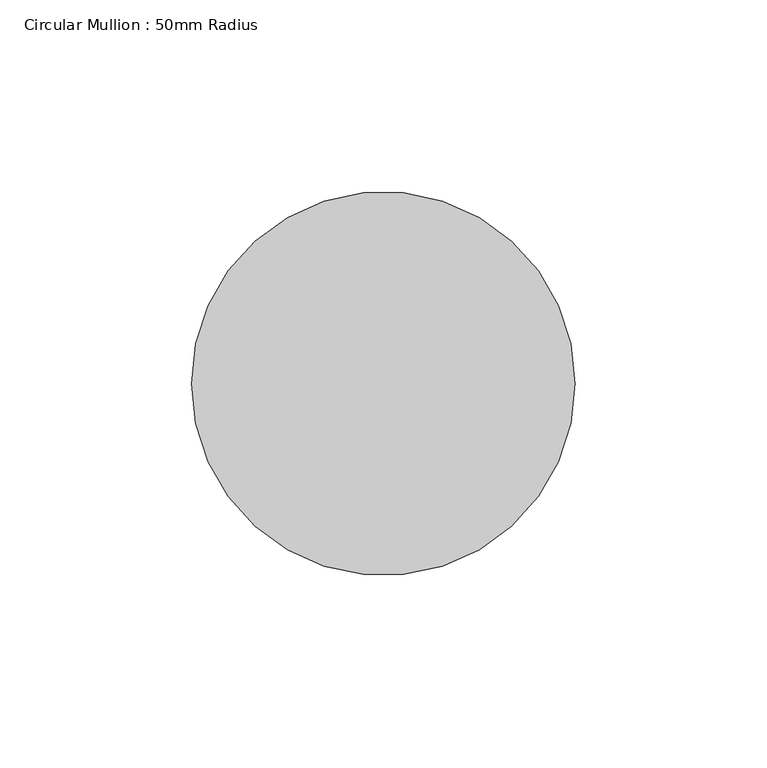
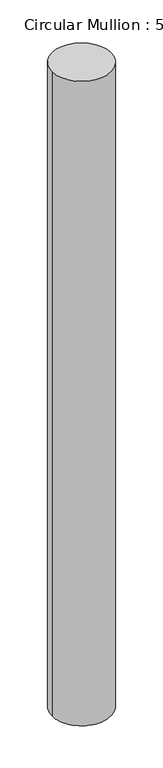
"""IFC4 building model written with IfcOpenShell, lengths in millimetres: member geometry, Circular Mullion : 50mm Radius."""

import ifcopenshell
import ifcopenshell.guid

model = None  # the IFC model being written
_history = None  # IfcOwnerHistory: only IFC2X3 demands one
_inside = {}  # id of a spatial element -> (the spatial element, [elements in it])
_under = {}  # id of a project, library or spatial element -> (it, [spatial elements below it])
_declared = {}  # id of a project -> (the project, [libraries it declares])
_typed = {}  # id of a type object -> (the type object, [elements of that type])
_made_of = {}  # id of a material, layer set ... -> (it, [elements and type objects made of it])


def new_model(schema):
    """Start an empty IFC model of exactly this schema.

    Asked for "IFC4X3", IfcOpenShell would pick the latest addendum, in which some entities
    have other attributes; the version numbers below select the first issue.
    IFC2X3 requires an IfcOwnerHistory on every rooted entity: one is made here for all.
    """
    global model, _history
    if schema == "IFC4X3":
        model = ifcopenshell.file(schema_version=(4, 3, 0, 0))
    else:
        model = ifcopenshell.file(schema=schema)
    _inside.clear()
    _under.clear()
    _declared.clear()
    _typed.clear()
    _made_of.clear()
    _history = None
    if model.schema == "IFC2X3":
        org = make("IfcOrganization", Name="unknown")
        user = make(
            "IfcPersonAndOrganization",
            ThePerson=make("IfcPerson", FamilyName="unknown"),
            TheOrganization=org,
        )
        app = make(
            "IfcApplication",
            ApplicationDeveloper=org,
            Version="unknown",
            ApplicationFullName="unknown",
            ApplicationIdentifier="unknown",
        )
        _history = make(
            "IfcOwnerHistory",
            OwningUser=user,
            OwningApplication=app,
            ChangeAction="ADDED",
            CreationDate=0,
        )
    return model


def make(cls, **values):
    """One entity of the class cls with the attributes given. An attribute that is None is left unset."""
    return model.create_entity(
        cls, **{name: value for name, value in values.items() if value is not None}
    )


def rooted(cls, **values):
    """An entity with a GlobalId (a new one), such as an element, a storey or a relation."""
    return make(cls, GlobalId=ifcopenshell.guid.new(), OwnerHistory=_history, **values)


def si_unit(unit_type, name, prefix=None):
    """IfcSIUnit, for example si_unit("LENGTHUNIT", "METRE", prefix="MILLI")."""
    return make("IfcSIUnit", UnitType=unit_type, Prefix=prefix, Name=name)


def assignment(units):
    """IfcUnitAssignment: the units of a project."""
    return None if units is None else make("IfcUnitAssignment", Units=units)


def point(xyz):
    """IfcCartesianPoint."""
    return None if xyz is None else make("IfcCartesianPoint", Coordinates=xyz)


def direction(xyz):
    """IfcDirection."""
    return None if xyz is None else make("IfcDirection", DirectionRatios=xyz)


def frame(location, z_axis=None, x_axis=None):
    """IfcAxis2Placement3D, a coordinate frame: its origin and axes. An axis left out is left unset."""
    return make(
        "IfcAxis2Placement3D",
        Location=point(location),
        Axis=direction(z_axis),
        RefDirection=direction(x_axis),
    )


def origin():
    """The frame at (0, 0, 0) with its axes left unset."""
    return frame((0.0, 0.0, 0.0))


def place(relative_to, where):
    """IfcLocalPlacement: puts the frame where relative to a parent placement (None: the world)."""
    return make(
        "IfcLocalPlacement", PlacementRelTo=relative_to, RelativePlacement=where
    )


def context(
    kind, dimensions, precision=None, world=None, true_north=None, identifier=None
):
    """IfcGeometricRepresentationContext, for example the 3D "Model" context."""
    return make(
        "IfcGeometricRepresentationContext",
        ContextIdentifier=identifier,
        ContextType=kind,
        CoordinateSpaceDimension=dimensions,
        Precision=precision,
        WorldCoordinateSystem=world,
        TrueNorth=true_north,
    )


def project(units=None, contexts=None):
    """IfcProject with its units and contexts."""
    return rooted(
        "IfcProject",
        Name="project",
        RepresentationContexts=contexts,
        UnitsInContext=assignment(units),
    )


def spatial(cls, under=None, at=None, **own):
    """A site, building, storey or space (cls), placed at a placement, below another one or the project."""
    s = rooted(cls, ObjectPlacement=at, **own)
    if under is not None:
        _under.setdefault(under.id(), (under, []))[1].append(s)
    return s


def ellipse_curve(where, semi_axis1, semi_axis2):
    """IfcEllipse in the frame where."""
    return make(
        "IfcEllipse", Position=where, SemiAxis1=semi_axis1, SemiAxis2=semi_axis2
    )


def shape(context_of_items, identifier, shape_type, items):
    """IfcShapeRepresentation: the items that make up one representation, for example the "Body"."""
    return make(
        "IfcShapeRepresentation",
        ContextOfItems=context_of_items,
        RepresentationIdentifier=identifier,
        RepresentationType=shape_type,
        Items=items,
    )


def source(mapping_origin, context_of_items, identifier, shape_type, items):
    """IfcRepresentationMap: a shape defined once, which mapped items show again and again."""
    return make(
        "IfcRepresentationMap",
        MappingOrigin=mapping_origin,
        MappedRepresentation=shape(context_of_items, identifier, shape_type, items),
    )


def transform(
    local_origin,
    x_axis=None,
    y_axis=None,
    z_axis=None,
    scale=None,
    scale2=None,
    scale3=None,
    uniform=True,
):
    """IfcCartesianTransformationOperator3D, or its non-uniform kind. x_axis, y_axis, z_axis: its Axis1, 2, 3."""
    if uniform:
        return make(
            "IfcCartesianTransformationOperator3D",
            Axis1=direction(x_axis),
            Axis2=direction(y_axis),
            LocalOrigin=point(local_origin),
            Scale=scale,
            Axis3=direction(z_axis),
        )
    return make(
        "IfcCartesianTransformationOperator3DnonUniform",
        Axis1=direction(x_axis),
        Axis2=direction(y_axis),
        LocalOrigin=point(local_origin),
        Scale=scale,
        Axis3=direction(z_axis),
        Scale2=scale2,
        Scale3=scale3,
    )


def mapped(mapping_source, mapping_target):
    """IfcMappedItem: shows the shape of a source again, moved by a transform."""
    return make(
        "IfcMappedItem", MappingSource=mapping_source, MappingTarget=mapping_target
    )


def made_of(thing, what):
    """Note that an element or type object is made of a material, layer set ...; save() writes the relation."""
    if what is not None:
        _made_of.setdefault(what.id(), (what, []))[1].append(thing)
    return thing


def element(
    cls,
    number,
    at=None,
    inside=None,
    cuts=None,
    type_object=None,
    material=None,
    context=None,
    identifier="Body",
    shape_type=None,
    held_by="IfcProductDefinitionShape",
    body=None,
    shapes=None,
    **own,
):
    """One element of the class cls, such as IfcWall. Its Tag is "e" and its number.

    at: its placement. inside: the storey or other place that contains it. cuts: it is an
    opening in that element (IfcRelVoidsElement). A single representation is given by context,
    identifier, shape_type and body (its items); several are given by shapes. held_by: the class
    of the entity that holds the representations. save() writes the other relations.
    """
    e = rooted(cls, Tag="e%d" % number, ObjectPlacement=at, **own)
    if body is not None:
        shapes = [shape(context, identifier, shape_type, body)]
    if shapes is not None:
        e.Representation = make(held_by, Representations=shapes)
    if inside is not None:
        _inside.setdefault(inside.id(), (inside, []))[1].append(e)
    if cuts is not None:
        rooted(
            "IfcRelVoidsElement", RelatingBuildingElement=cuts, RelatedOpeningElement=e
        )
    if type_object is not None:
        _typed.setdefault(type_object.id(), (type_object, []))[1].append(e)
    return made_of(e, material)


def aggregate(whole, parts):
    """IfcRelAggregates: a whole, such as a stair, and the parts it consists of."""
    return rooted("IfcRelAggregates", RelatingObject=whole, RelatedObjects=parts)


def save(model, path):
    """Write the relations noted so far, then the file.

    IfcRelAggregates (storeys below a building ...), IfcRelContainedInSpatialStructure (elements
    in a storey), IfcRelDefinesByType, IfcRelAssociatesMaterial and IfcRelDeclares: one each for
    every whole, place, type object, material and project.
    """
    for whole, parts in _under.values():
        aggregate(whole, parts)
    for where, things in _inside.values():
        rooted(
            "IfcRelContainedInSpatialStructure",
            RelatedElements=things,
            RelatingStructure=where,
        )
    for kind, things in _typed.values():
        rooted("IfcRelDefinesByType", RelatedObjects=things, RelatingType=kind)
    for what, things in _made_of.values():
        rooted("IfcRelAssociatesMaterial", RelatedObjects=things, RelatingMaterial=what)
    for by, libraries in _declared.values():
        rooted("IfcRelDeclares", RelatingContext=by, RelatedDefinitions=libraries)
    model.write(path)


def plane_surface(at):
    """IfcPlane: the flat surface through the origin of the frame at, square to its z axis."""
    return make("IfcPlane", Position=at)


def cylinder_surface(at, radius):
    """IfcCylindricalSurface: all points at the distance radius from the z axis of the frame at."""
    return make("IfcCylindricalSurface", Position=at, Radius=radius)


def advanced_brep(points, edges, surfaces, faces):
    """IfcAdvancedBrep: a solid bounded by faces that lie on surfaces and meet in shared edges.

    An edge is (start, end): straight between two places in points (the first is 0);
    or (start, end, curve); or (start, end, curve, False) where it runs against its curve.
    A face is (place in surfaces, loops), or (place, loops, False) where it looks against
    its surface's normal. A loop lists edges by number (the first is 1), with a minus sign
    where the edge is run from its end to its start. The first loop is the outer one.
    """
    corners = [point(p) for p in points]
    vertices = [make("IfcVertexPoint", VertexGeometry=c) for c in corners]
    made = []
    for start, end, *more in edges:
        made.append(
            make(
                "IfcEdgeCurve",
                EdgeStart=vertices[start],
                EdgeEnd=vertices[end],
                EdgeGeometry=more[0] if more else make("IfcPolyline", Points=[corners[start], corners[end]]),
                SameSense=more[1] if len(more) > 1 else True,
            )
        )
    hull = []
    for where, loops, *sense in faces:
        bounds = []
        for j, loop in enumerate(loops):
            ring = [make("IfcOrientedEdge", EdgeElement=made[abs(k) - 1], Orientation=k > 0) for k in loop]
            bounds.append(
                make(
                    "IfcFaceOuterBound" if j == 0 else "IfcFaceBound",
                    Bound=make("IfcEdgeLoop", EdgeList=ring),
                    Orientation=True,
                )
            )
        hull.append(make("IfcAdvancedFace", Bounds=bounds, FaceSurface=surfaces[where], SameSense=sense[0] if sense else True))
    return make("IfcAdvancedBrep", Outer=make("IfcClosedShell", CfsFaces=hull))


def circular_mullion_50mm_radius_71162de6(model_context):
    return source(origin(), model_context, "Body", "AdvancedBrep", [
        advanced_brep(
        [(-100.0, 0.0, 0.9449858), (0.0, 0.0, 0.0), (0.0, 0.0, -1144.6892863), (-100.0, 0.0, -1145.6702895)],
        [
            (0, 1, ellipse_curve(frame((-50.0, 0.0, 0.4724929), z_axis=(-0.009448458751315407, -0.014383764193855156, -0.9998519060115054), x_axis=(-0.548945231973302, -0.8356811391006849, 0.017209475446963905)), 50.0074058, 50.0)),
            (1, 2),
            (2, 3, ellipse_curve(frame((-50.0, 0.0, -1145.1797879), z_axis=(-0.009808466948255391, -0.014931818977067286, 0.9998404046437417), x_axis=(0.5489389174171557, 0.8356715262009603, 0.017865196383996137)), 50.007981, 50.0)),
            (3, 0),
            (1, 0, ellipse_curve(frame((-50.0, 0.0, 0.4724929), z_axis=(-0.009448458751315407, -0.014383764193855156, -0.9998519060115054), x_axis=(-0.548945231973302, -0.8356811391006849, 0.017209475446963905)), 50.0074058, 50.0)),
            (3, 2, ellipse_curve(frame((-50.0, 0.0, -1145.1797879), z_axis=(-0.009808466948255391, -0.014931818977067286, 0.9998404046437417), x_axis=(0.5489389174171557, 0.8356715262009603, 0.017865196383996137)), 50.007981, 50.0)),
        ],
        [
            cylinder_surface(frame((-50.0, 0.0, 0.0), z_axis=(0.0, 0.0, 1.0), x_axis=(1.0, 0.0, 0.0)), 50.0),
            plane_surface(frame((-254.7533386, 167.3432892, 0.0), z_axis=(0.009448458751315409, 0.01438376419385516, 0.9998519060115056), x_axis=(0.5489452319733018, 0.835681139100685, -0.017209475446966372))),
            plane_surface(frame((-254.7533386, 167.3432892, -1144.6892863), z_axis=(0.009808466948255393, 0.01493181897706729, -0.9998404046437419), x_axis=(0.5489389174171557, 0.8356715262009604, 0.01786519638400108))),
        ],
        [
            (0, [[1, 2, 3, 4]]),
            (0, [[5, -4, 6, -2]]),
            (1, [[-1, -5]]),
            (2, [[-6, -3]]),
        ],
    ),
    ])


if __name__ == "__main__":
    model = new_model("IFC4")
    model_context = context("Model", 3, world=origin())
    ifc_project = project(units=[si_unit("LENGTHUNIT", "METRE", prefix="MILLI")], contexts=[model_context])
    site = spatial("IfcSite", under=ifc_project)
    building = spatial("IfcBuilding", under=site)
    placement = place(None, origin())
    circular_mullion_50mm_radius_shape = circular_mullion_50mm_radius_71162de6(model_context)
    element("IfcMember", 1, ObjectType="Circular Mullion : 50mm Radius", at=placement, inside=building, context=model_context, shape_type="MappedRepresentation", body=[
        mapped(circular_mullion_50mm_radius_shape, transform((0.0, 0.0, 0.0), x_axis=(1.0, 0.0, 0.0), y_axis=(0.0, 1.0, 0.0), z_axis=(0.0, 0.0, 1.0))),
    ])
    save(model, "model.ifc")

# Revit data of these elements
# Type "Circular Mullion : 50mm Radius"
#   built-in parameter 1007350 = 0.164042 (stored number, unit not read)
# Element 1 (IfcMember, "Circular Mullion : 50mm Radius")
#   Materials on its faces: "Aluminium"
# Materials
#   "Aluminium": class "Metal", colour RGB 247 247 247, transparency 0, Description = "Aluminium 6061", Cost = 0
